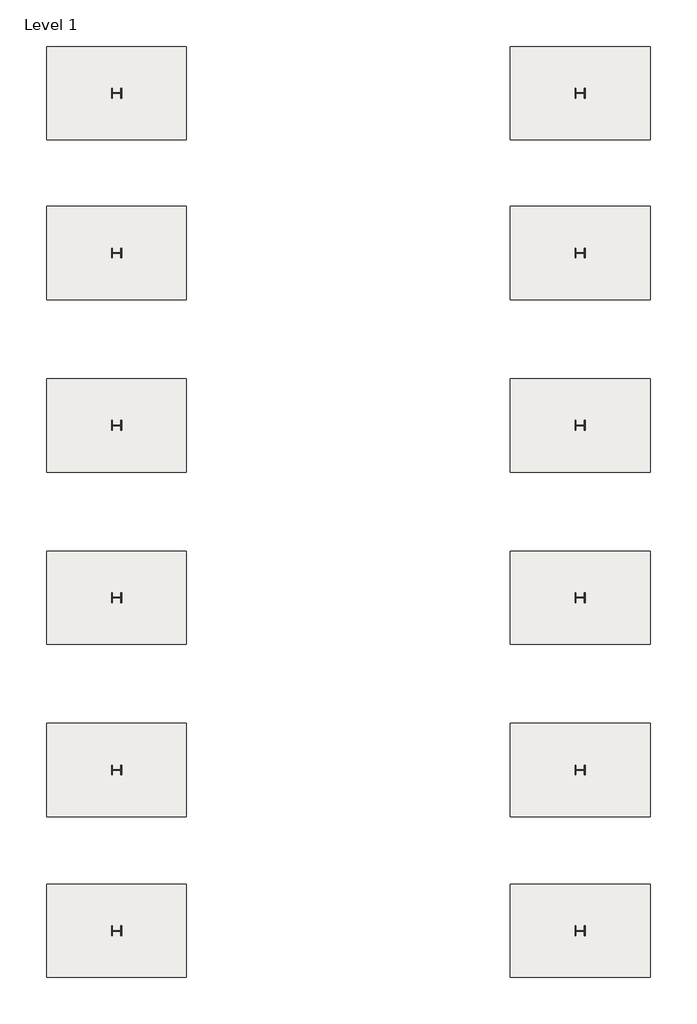
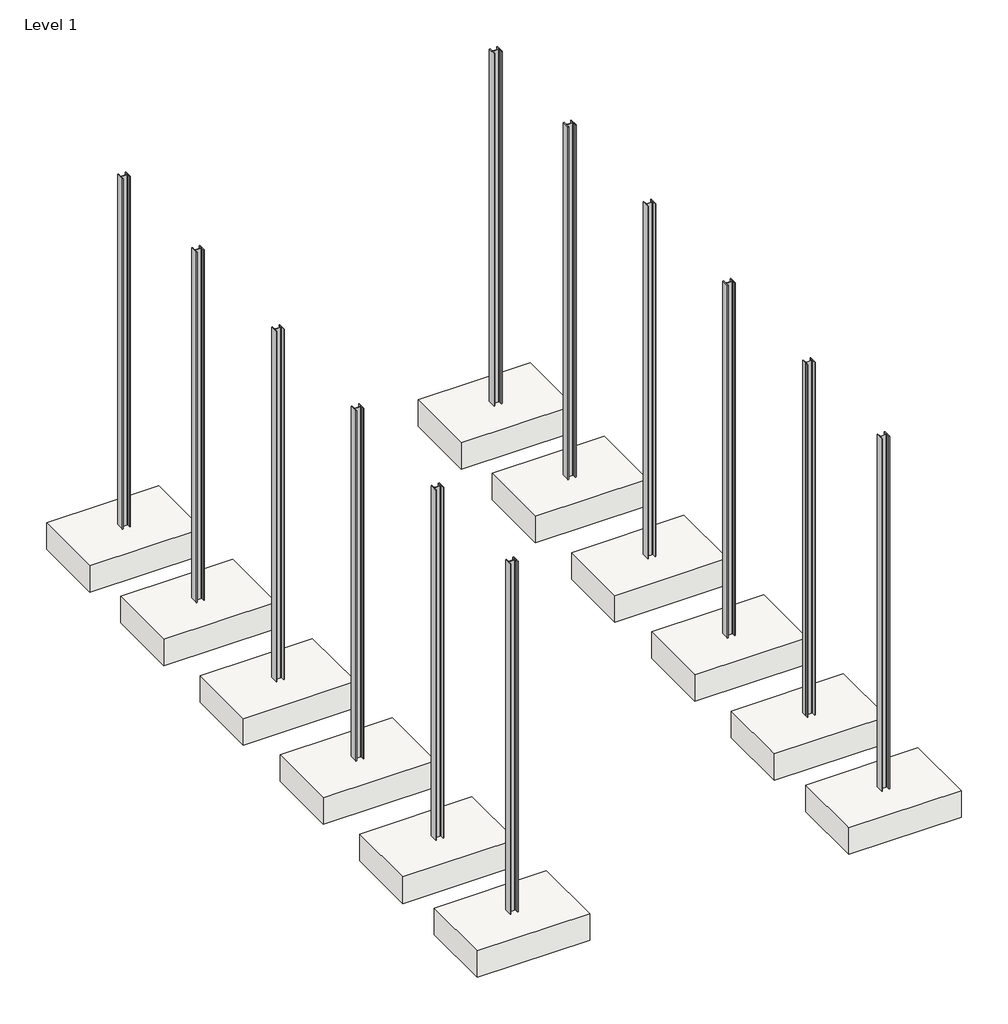
# One storey: 12 columns, 12 slabs.
"""IFC4 building model written with IfcOpenShell, lengths in millimetres."""

import ifcopenshell
import ifcopenshell.guid

model = None  # the IFC model being written
_history = None  # IfcOwnerHistory: only IFC2X3 demands one
_inside = {}  # id of a spatial element -> (the spatial element, [elements in it])
_under = {}  # id of a project, library or spatial element -> (it, [spatial elements below it])
_declared = {}  # id of a project -> (the project, [libraries it declares])
_typed = {}  # id of a type object -> (the type object, [elements of that type])
_made_of = {}  # id of a material, layer set ... -> (it, [elements and type objects made of it])


def new_model(schema):
    """Start an empty IFC model of exactly this schema.

    Asked for "IFC4X3", IfcOpenShell would pick the latest addendum, in which some entities
    have other attributes; the version numbers below select the first issue.
    IFC2X3 requires an IfcOwnerHistory on every rooted entity: one is made here for all.
    """
    global model, _history
    if schema == "IFC4X3":
        model = ifcopenshell.file(schema_version=(4, 3, 0, 0))
    else:
        model = ifcopenshell.file(schema=schema)
    _inside.clear()
    _under.clear()
    _declared.clear()
    _typed.clear()
    _made_of.clear()
    _history = None
    if model.schema == "IFC2X3":
        org = make("IfcOrganization", Name="unknown")
        user = make(
            "IfcPersonAndOrganization",
            ThePerson=make("IfcPerson", FamilyName="unknown"),
            TheOrganization=org,
        )
        app = make(
            "IfcApplication",
            ApplicationDeveloper=org,
            Version="unknown",
            ApplicationFullName="unknown",
            ApplicationIdentifier="unknown",
        )
        _history = make(
            "IfcOwnerHistory",
            OwningUser=user,
            OwningApplication=app,
            ChangeAction="ADDED",
            CreationDate=0,
        )
    return model


def make(cls, **values):
    """One entity of the class cls with the attributes given. An attribute that is None is left unset."""
    return model.create_entity(
        cls, **{name: value for name, value in values.items() if value is not None}
    )


def rooted(cls, **values):
    """An entity with a GlobalId (a new one), such as an element, a storey or a relation."""
    return make(cls, GlobalId=ifcopenshell.guid.new(), OwnerHistory=_history, **values)


def si_unit(unit_type, name, prefix=None):
    """IfcSIUnit, for example si_unit("LENGTHUNIT", "METRE", prefix="MILLI")."""
    return make("IfcSIUnit", UnitType=unit_type, Prefix=prefix, Name=name)


def assignment(units):
    """IfcUnitAssignment: the units of a project."""
    return None if units is None else make("IfcUnitAssignment", Units=units)


def point(xyz):
    """IfcCartesianPoint."""
    return None if xyz is None else make("IfcCartesianPoint", Coordinates=xyz)


def direction(xyz):
    """IfcDirection."""
    return None if xyz is None else make("IfcDirection", DirectionRatios=xyz)


def frame(location, z_axis=None, x_axis=None):
    """IfcAxis2Placement3D, a coordinate frame: its origin and axes. An axis left out is left unset."""
    return make(
        "IfcAxis2Placement3D",
        Location=point(location),
        Axis=direction(z_axis),
        RefDirection=direction(x_axis),
    )


def frame_2d(location, x_axis=None):
    """IfcAxis2Placement2D, a coordinate frame in the plane: its origin and x axis."""
    return make(
        "IfcAxis2Placement2D", Location=point(location), RefDirection=direction(x_axis)
    )


def origin():
    """The frame at (0, 0, 0) with its axes left unset."""
    return frame((0.0, 0.0, 0.0))


def place(relative_to, where):
    """IfcLocalPlacement: puts the frame where relative to a parent placement (None: the world)."""
    return make(
        "IfcLocalPlacement", PlacementRelTo=relative_to, RelativePlacement=where
    )


def context(
    kind, dimensions, precision=None, world=None, true_north=None, identifier=None
):
    """IfcGeometricRepresentationContext, for example the 3D "Model" context."""
    return make(
        "IfcGeometricRepresentationContext",
        ContextIdentifier=identifier,
        ContextType=kind,
        CoordinateSpaceDimension=dimensions,
        Precision=precision,
        WorldCoordinateSystem=world,
        TrueNorth=true_north,
    )


def project(units=None, contexts=None):
    """IfcProject with its units and contexts."""
    return rooted(
        "IfcProject",
        Name="project",
        RepresentationContexts=contexts,
        UnitsInContext=assignment(units),
    )


def spatial(cls, under=None, at=None, **own):
    """A site, building, storey or space (cls), placed at a placement, below another one or the project."""
    s = rooted(cls, ObjectPlacement=at, **own)
    if under is not None:
        _under.setdefault(under.id(), (under, []))[1].append(s)
    return s


def polyline(points):
    """IfcPolyline through the points."""
    return make("IfcPolyline", Points=[point(p) for p in points])


def circle_curve(where, radius):
    """IfcCircle in the frame where."""
    return make("IfcCircle", Position=where, Radius=radius)


def trimmed(basis, trim1, trim2, sense, master):
    """IfcTrimmedCurve: the piece of a basis curve between two trims."""
    return make(
        "IfcTrimmedCurve",
        BasisCurve=basis,
        Trim1=trim1,
        Trim2=trim2,
        SenseAgreement=sense,
        MasterRepresentation=master,
    )


def segment(curve, same_sense, transition):
    """IfcCompositeCurveSegment."""
    return make(
        "IfcCompositeCurveSegment",
        Transition=transition,
        SameSense=same_sense,
        ParentCurve=curve,
    )


def composite_curve(segments, self_intersect=None):
    """IfcCompositeCurve: segments joined end to end."""
    return make("IfcCompositeCurve", Segments=segments, SelfIntersect=self_intersect)


def outline(outer, holes=None, kind="AREA"):
    """IfcArbitraryClosedProfileDef: a profile drawn as a closed curve; with holes, ...WithVoids."""
    if holes is None:
        return make("IfcArbitraryClosedProfileDef", ProfileType=kind, OuterCurve=outer)
    return make(
        "IfcArbitraryProfileDefWithVoids",
        ProfileType=kind,
        OuterCurve=outer,
        InnerCurves=holes,
    )


def extrude(swept, where, along, depth):
    """IfcExtrudedAreaSolid: the profile swept, set in the frame where, extruded along a direction by depth."""
    return make(
        "IfcExtrudedAreaSolid",
        SweptArea=swept,
        Position=where,
        ExtrudedDirection=direction(along),
        Depth=depth,
    )


def shape(context_of_items, identifier, shape_type, items):
    """IfcShapeRepresentation: the items that make up one representation, for example the "Body"."""
    return make(
        "IfcShapeRepresentation",
        ContextOfItems=context_of_items,
        RepresentationIdentifier=identifier,
        RepresentationType=shape_type,
        Items=items,
    )


def source(mapping_origin, context_of_items, identifier, shape_type, items):
    """IfcRepresentationMap: a shape defined once, which mapped items show again and again."""
    return make(
        "IfcRepresentationMap",
        MappingOrigin=mapping_origin,
        MappedRepresentation=shape(context_of_items, identifier, shape_type, items),
    )


def transform(
    local_origin,
    x_axis=None,
    y_axis=None,
    z_axis=None,
    scale=None,
    scale2=None,
    scale3=None,
    uniform=True,
):
    """IfcCartesianTransformationOperator3D, or its non-uniform kind. x_axis, y_axis, z_axis: its Axis1, 2, 3."""
    if uniform:
        return make(
            "IfcCartesianTransformationOperator3D",
            Axis1=direction(x_axis),
            Axis2=direction(y_axis),
            LocalOrigin=point(local_origin),
            Scale=scale,
            Axis3=direction(z_axis),
        )
    return make(
        "IfcCartesianTransformationOperator3DnonUniform",
        Axis1=direction(x_axis),
        Axis2=direction(y_axis),
        LocalOrigin=point(local_origin),
        Scale=scale,
        Axis3=direction(z_axis),
        Scale2=scale2,
        Scale3=scale3,
    )


def mapped(mapping_source, mapping_target):
    """IfcMappedItem: shows the shape of a source again, moved by a transform."""
    return make(
        "IfcMappedItem", MappingSource=mapping_source, MappingTarget=mapping_target
    )


def made_of(thing, what):
    """Note that an element or type object is made of a material, layer set ...; save() writes the relation."""
    if what is not None:
        _made_of.setdefault(what.id(), (what, []))[1].append(thing)
    return thing


def element(
    cls,
    number,
    at=None,
    inside=None,
    cuts=None,
    type_object=None,
    material=None,
    context=None,
    identifier="Body",
    shape_type=None,
    held_by="IfcProductDefinitionShape",
    body=None,
    shapes=None,
    **own,
):
    """One element of the class cls, such as IfcWall. Its Tag is "e" and its number.

    at: its placement. inside: the storey or other place that contains it. cuts: it is an
    opening in that element (IfcRelVoidsElement). A single representation is given by context,
    identifier, shape_type and body (its items); several are given by shapes. held_by: the class
    of the entity that holds the representations. save() writes the other relations.
    """
    e = rooted(cls, Tag="e%d" % number, ObjectPlacement=at, **own)
    if body is not None:
        shapes = [shape(context, identifier, shape_type, body)]
    if shapes is not None:
        e.Representation = make(held_by, Representations=shapes)
    if inside is not None:
        _inside.setdefault(inside.id(), (inside, []))[1].append(e)
    if cuts is not None:
        rooted(
            "IfcRelVoidsElement", RelatingBuildingElement=cuts, RelatedOpeningElement=e
        )
    if type_object is not None:
        _typed.setdefault(type_object.id(), (type_object, []))[1].append(e)
    return made_of(e, material)


def aggregate(whole, parts):
    """IfcRelAggregates: a whole, such as a stair, and the parts it consists of."""
    return rooted("IfcRelAggregates", RelatingObject=whole, RelatedObjects=parts)


def save(model, path):
    """Write the relations noted so far, then the file.

    IfcRelAggregates (storeys below a building ...), IfcRelContainedInSpatialStructure (elements
    in a storey), IfcRelDefinesByType, IfcRelAssociatesMaterial and IfcRelDeclares: one each for
    every whole, place, type object, material and project.
    """
    for whole, parts in _under.values():
        aggregate(whole, parts)
    for where, things in _inside.values():
        rooted(
            "IfcRelContainedInSpatialStructure",
            RelatedElements=things,
            RelatingStructure=where,
        )
    for kind, things in _typed.values():
        rooted("IfcRelDefinesByType", RelatedObjects=things, RelatingType=kind)
    for what, things in _made_of.values():
        rooted("IfcRelAssociatesMaterial", RelatedObjects=things, RelatingMaterial=what)
    for by, libraries in _declared.values():
        rooted("IfcRelDeclares", RelatingContext=by, RelatedDefinitions=libraries)
    model.write(path)


def slab_5ba74754(model_context):
    return source(origin(), model_context, "Body", "SweptSolid", [
        extrude(outline(polyline([(609.6, 914.4), (609.6, -914.4), (-609.6, -914.4), (-609.6, 914.4), (609.6, 914.4)])), frame((0.0, 0.0, -457.2), z_axis=(0.0, 0.0, 1.0), x_axis=(1.0, 0.0, 0.0)), (0.0, 0.0, 1.0), 457.2),
    ])


model = new_model("IFC4")

# Units and contexts
model_context = context("Model", 3, world=origin())
ifc_project = project(units=[si_unit("LENGTHUNIT", "METRE", prefix="MILLI")], contexts=[model_context])

# Site, building, storey
site = spatial("IfcSite", under=ifc_project)
building = spatial("IfcBuilding", under=site)
storey = spatial("IfcBuildingStorey", under=building, Name="Level 1", Elevation=0.0)

# Columns
placement = place(None, origin())
element("IfcColumn", 1, ObjectType="W-Wide Flange-Column : W5X19", at=placement, inside=storey, context=model_context, shape_type="SweptSolid", body=[
    extrude(outline(composite_curve([segment(polyline([(-222.2451664, 2315.5517583), (-211.3231664, 2315.5517583), (-211.3231664, 2264.8152583)]), True, "CONTINUOUS"), segment(trimmed(circle_curve(frame_2d((-201.6076664, 2264.8152583)), 9.7155), [point((-211.3231664, 2264.8152583))], [point((-201.6076664, 2255.0997583))], True, "CARTESIAN"), True, "CONTINUOUS"), segment(polyline([(-201.6076664, 2255.0997583), (-112.0726664, 2255.0997583)]), True, "CONTINUOUS"), segment(trimmed(circle_curve(frame_2d((-112.0726664, 2264.8152583)), 9.7155), [point((-112.0726664, 2255.0997583))], [point((-102.3571664, 2264.8152583))], True, "CARTESIAN"), True, "CONTINUOUS"), segment(polyline([(-102.3571664, 2264.8152583), (-102.3571664, 2315.5517583), (-91.4351664, 2315.5517583), (-91.4351664, 2187.7897583), (-102.3571664, 2187.7897583), (-102.3571664, 2238.5262583)]), True, "CONTINUOUS"), segment(trimmed(circle_curve(frame_2d((-112.0726664, 2238.5262583)), 9.7155), [point((-102.3571664, 2238.5262583))], [point((-112.0726664, 2248.2417583))], True, "CARTESIAN"), True, "CONTINUOUS"), segment(polyline([(-112.0726664, 2248.2417583), (-201.6076664, 2248.2417583)]), True, "CONTINUOUS"), segment(trimmed(circle_curve(frame_2d((-201.6076664, 2238.5262583)), 9.7155), [point((-201.6076664, 2248.2417583))], [point((-211.3231664, 2238.5262583))], True, "CARTESIAN"), True, "CONTINUOUS"), segment(polyline([(-211.3231664, 2238.5262583), (-211.3231664, 2187.7897583), (-222.2451664, 2187.7897583), (-222.2451664, 2315.5517583)]), True, "CONTINUOUS")], self_intersect=False)), frame((0.0, 0.0, -304.8), z_axis=(0.0, 0.0, 1.0), x_axis=(1.0, 0.0, 0.0)), (0.0, 0.0, 1.0), 6079.1336143),
])
element("IfcColumn", 2, ObjectType="W-Wide Flange-Column : W5X19", at=placement, inside=storey, context=model_context, shape_type="SweptSolid", body=[
    extrude(outline(composite_curve([segment(polyline([(-6280.1451664, 2315.5517583), (-6269.2231664, 2315.5517583), (-6269.2231664, 2264.8152583)]), True, "CONTINUOUS"), segment(trimmed(circle_curve(frame_2d((-6259.5076664, 2264.8152583)), 9.7155), [point((-6269.2231664, 2264.8152583))], [point((-6259.5076664, 2255.0997583))], True, "CARTESIAN"), True, "CONTINUOUS"), segment(polyline([(-6259.5076664, 2255.0997583), (-6169.9726664, 2255.0997583)]), True, "CONTINUOUS"), segment(trimmed(circle_curve(frame_2d((-6169.9726664, 2264.8152583)), 9.7155), [point((-6169.9726664, 2255.0997583))], [point((-6160.2571664, 2264.8152583))], True, "CARTESIAN"), True, "CONTINUOUS"), segment(polyline([(-6160.2571664, 2264.8152583), (-6160.2571664, 2315.5517583), (-6149.3351664, 2315.5517583), (-6149.3351664, 2187.7897583), (-6160.2571664, 2187.7897583), (-6160.2571664, 2238.5262583)]), True, "CONTINUOUS"), segment(trimmed(circle_curve(frame_2d((-6169.9726664, 2238.5262583)), 9.7155), [point((-6160.2571664, 2238.5262583))], [point((-6169.9726664, 2248.2417583))], True, "CARTESIAN"), True, "CONTINUOUS"), segment(polyline([(-6169.9726664, 2248.2417583), (-6259.5076664, 2248.2417583)]), True, "CONTINUOUS"), segment(trimmed(circle_curve(frame_2d((-6259.5076664, 2238.5262583)), 9.7155), [point((-6259.5076664, 2248.2417583))], [point((-6269.2231664, 2238.5262583))], True, "CARTESIAN"), True, "CONTINUOUS"), segment(polyline([(-6269.2231664, 2238.5262583), (-6269.2231664, 2187.7897583), (-6280.1451664, 2187.7897583), (-6280.1451664, 2315.5517583)]), True, "CONTINUOUS")], self_intersect=False)), frame((0.0, 0.0, -304.8), z_axis=(0.0, 0.0, 1.0), x_axis=(1.0, 0.0, 0.0)), (0.0, 0.0, 1.0), 6040.3114063),
])
element("IfcColumn", 3, ObjectType="W-Wide Flange-Column : W5X19", at=placement, inside=storey, context=model_context, shape_type="SweptSolid", body=[
    extrude(outline(composite_curve([segment(polyline([(-222.2451664, 4567.4626058), (-211.3231664, 4567.4626058), (-211.3231664, 4516.7261058)]), True, "CONTINUOUS"), segment(trimmed(circle_curve(frame_2d((-201.6076664, 4516.7261058)), 9.7155), [point((-211.3231664, 4516.7261058))], [point((-201.6076664, 4507.0106058))], True, "CARTESIAN"), True, "CONTINUOUS"), segment(polyline([(-201.6076664, 4507.0106058), (-112.0726664, 4507.0106058)]), True, "CONTINUOUS"), segment(trimmed(circle_curve(frame_2d((-112.0726664, 4516.7261058)), 9.7155), [point((-112.0726664, 4507.0106058))], [point((-102.3571664, 4516.7261058))], True, "CARTESIAN"), True, "CONTINUOUS"), segment(polyline([(-102.3571664, 4516.7261058), (-102.3571664, 4567.4626058), (-91.4351664, 4567.4626058), (-91.4351664, 4439.7006058), (-102.3571664, 4439.7006058), (-102.3571664, 4490.4371058)]), True, "CONTINUOUS"), segment(trimmed(circle_curve(frame_2d((-112.0726664, 4490.4371058)), 9.7155), [point((-102.3571664, 4490.4371058))], [point((-112.0726664, 4500.1526058))], True, "CARTESIAN"), True, "CONTINUOUS"), segment(polyline([(-112.0726664, 4500.1526058), (-201.6076664, 4500.1526058)]), True, "CONTINUOUS"), segment(trimmed(circle_curve(frame_2d((-201.6076664, 4490.4371058)), 9.7155), [point((-201.6076664, 4500.1526058))], [point((-211.3231664, 4490.4371058))], True, "CARTESIAN"), True, "CONTINUOUS"), segment(polyline([(-211.3231664, 4490.4371058), (-211.3231664, 4439.7006058), (-222.2451664, 4439.7006058), (-222.2451664, 4567.4626058)]), True, "CONTINUOUS")], self_intersect=False)), frame((0.0, 0.0, -304.8), z_axis=(0.0, 0.0, 1.0), x_axis=(1.0, 0.0, 0.0)), (0.0, 0.0, 1.0), 6079.1336143),
])
element("IfcColumn", 4, ObjectType="W-Wide Flange-Column : W5X19", at=placement, inside=storey, context=model_context, shape_type="SweptSolid", body=[
    extrude(outline(composite_curve([segment(polyline([(-6280.1451664, 4567.4626058), (-6269.2231664, 4567.4626058), (-6269.2231664, 4516.7261058)]), True, "CONTINUOUS"), segment(trimmed(circle_curve(frame_2d((-6259.5076664, 4516.7261058)), 9.7155), [point((-6269.2231664, 4516.7261058))], [point((-6259.5076664, 4507.0106058))], True, "CARTESIAN"), True, "CONTINUOUS"), segment(polyline([(-6259.5076664, 4507.0106058), (-6169.9726664, 4507.0106058)]), True, "CONTINUOUS"), segment(trimmed(circle_curve(frame_2d((-6169.9726664, 4516.7261058)), 9.7155), [point((-6169.9726664, 4507.0106058))], [point((-6160.2571664, 4516.7261058))], True, "CARTESIAN"), True, "CONTINUOUS"), segment(polyline([(-6160.2571664, 4516.7261058), (-6160.2571664, 4567.4626058), (-6149.3351664, 4567.4626058), (-6149.3351664, 4439.7006058), (-6160.2571664, 4439.7006058), (-6160.2571664, 4490.4371058)]), True, "CONTINUOUS"), segment(trimmed(circle_curve(frame_2d((-6169.9726664, 4490.4371058)), 9.7155), [point((-6160.2571664, 4490.4371058))], [point((-6169.9726664, 4500.1526058))], True, "CARTESIAN"), True, "CONTINUOUS"), segment(polyline([(-6169.9726664, 4500.1526058), (-6259.5076664, 4500.1526058)]), True, "CONTINUOUS"), segment(trimmed(circle_curve(frame_2d((-6259.5076664, 4490.4371058)), 9.7155), [point((-6259.5076664, 4500.1526058))], [point((-6269.2231664, 4490.4371058))], True, "CARTESIAN"), True, "CONTINUOUS"), segment(polyline([(-6269.2231664, 4490.4371058), (-6269.2231664, 4439.7006058), (-6280.1451664, 4439.7006058), (-6280.1451664, 4567.4626058)]), True, "CONTINUOUS")], self_intersect=False)), frame((0.0, 0.0, -304.8), z_axis=(0.0, 0.0, 1.0), x_axis=(1.0, 0.0, 0.0)), (0.0, 0.0, 1.0), 6040.3114063),
])
element("IfcColumn", 5, ObjectType="W-Wide Flange-Column : W5X19", at=placement, inside=storey, context=model_context, shape_type="SweptSolid", body=[
    extrude(outline(composite_curve([segment(polyline([(-222.2451664, 6819.3734532), (-211.3231664, 6819.3734532), (-211.3231664, 6768.6369532)]), True, "CONTINUOUS"), segment(trimmed(circle_curve(frame_2d((-201.6076664, 6768.6369532)), 9.7155), [point((-211.3231664, 6768.6369532))], [point((-201.6076664, 6758.9214532))], True, "CARTESIAN"), True, "CONTINUOUS"), segment(polyline([(-201.6076664, 6758.9214532), (-112.0726664, 6758.9214532)]), True, "CONTINUOUS"), segment(trimmed(circle_curve(frame_2d((-112.0726664, 6768.6369532)), 9.7155), [point((-112.0726664, 6758.9214532))], [point((-102.3571664, 6768.6369532))], True, "CARTESIAN"), True, "CONTINUOUS"), segment(polyline([(-102.3571664, 6768.6369532), (-102.3571664, 6819.3734532), (-91.4351664, 6819.3734532), (-91.4351664, 6691.6114532), (-102.3571664, 6691.6114532), (-102.3571664, 6742.3479532)]), True, "CONTINUOUS"), segment(trimmed(circle_curve(frame_2d((-112.0726664, 6742.3479532)), 9.7155), [point((-102.3571664, 6742.3479532))], [point((-112.0726664, 6752.0634532))], True, "CARTESIAN"), True, "CONTINUOUS"), segment(polyline([(-112.0726664, 6752.0634532), (-201.6076664, 6752.0634532)]), True, "CONTINUOUS"), segment(trimmed(circle_curve(frame_2d((-201.6076664, 6742.3479532)), 9.7155), [point((-201.6076664, 6752.0634532))], [point((-211.3231664, 6742.3479532))], True, "CARTESIAN"), True, "CONTINUOUS"), segment(polyline([(-211.3231664, 6742.3479532), (-211.3231664, 6691.6114532), (-222.2451664, 6691.6114532), (-222.2451664, 6819.3734532)]), True, "CONTINUOUS")], self_intersect=False)), frame((0.0, 0.0, -304.8), z_axis=(0.0, 0.0, 1.0), x_axis=(1.0, 0.0, 0.0)), (0.0, 0.0, 1.0), 6079.1336143),
])
element("IfcColumn", 6, ObjectType="W-Wide Flange-Column : W5X19", at=placement, inside=storey, context=model_context, shape_type="SweptSolid", body=[
    extrude(outline(composite_curve([segment(polyline([(-6280.1451664, 6819.3734532), (-6269.2231664, 6819.3734532), (-6269.2231664, 6768.6369532)]), True, "CONTINUOUS"), segment(trimmed(circle_curve(frame_2d((-6259.5076664, 6768.6369532)), 9.7155), [point((-6269.2231664, 6768.6369532))], [point((-6259.5076664, 6758.9214532))], True, "CARTESIAN"), True, "CONTINUOUS"), segment(polyline([(-6259.5076664, 6758.9214532), (-6169.9726664, 6758.9214532)]), True, "CONTINUOUS"), segment(trimmed(circle_curve(frame_2d((-6169.9726664, 6768.6369532)), 9.7155), [point((-6169.9726664, 6758.9214532))], [point((-6160.2571664, 6768.6369532))], True, "CARTESIAN"), True, "CONTINUOUS"), segment(polyline([(-6160.2571664, 6768.6369532), (-6160.2571664, 6819.3734532), (-6149.3351664, 6819.3734532), (-6149.3351664, 6691.6114532), (-6160.2571664, 6691.6114532), (-6160.2571664, 6742.3479532)]), True, "CONTINUOUS"), segment(trimmed(circle_curve(frame_2d((-6169.9726664, 6742.3479532)), 9.7155), [point((-6160.2571664, 6742.3479532))], [point((-6169.9726664, 6752.0634532))], True, "CARTESIAN"), True, "CONTINUOUS"), segment(polyline([(-6169.9726664, 6752.0634532), (-6259.5076664, 6752.0634532)]), True, "CONTINUOUS"), segment(trimmed(circle_curve(frame_2d((-6259.5076664, 6742.3479532)), 9.7155), [point((-6259.5076664, 6752.0634532))], [point((-6269.2231664, 6742.3479532))], True, "CARTESIAN"), True, "CONTINUOUS"), segment(polyline([(-6269.2231664, 6742.3479532), (-6269.2231664, 6691.6114532), (-6280.1451664, 6691.6114532), (-6280.1451664, 6819.3734532)]), True, "CONTINUOUS")], self_intersect=False)), frame((0.0, 0.0, -304.8), z_axis=(0.0, 0.0, 1.0), x_axis=(1.0, 0.0, 0.0)), (0.0, 0.0, 1.0), 6040.3114063),
])
element("IfcColumn", 7, ObjectType="W-Wide Flange-Column : W5X19", at=placement, inside=storey, context=model_context, shape_type="SweptSolid", body=[
    extrude(outline(composite_curve([segment(polyline([(-222.2451664, 9071.2843006), (-211.3231664, 9071.2843006), (-211.3231664, 9020.5478006)]), True, "CONTINUOUS"), segment(trimmed(circle_curve(frame_2d((-201.6076664, 9020.5478006)), 9.7155), [point((-211.3231664, 9020.5478006))], [point((-201.6076664, 9010.8323006))], True, "CARTESIAN"), True, "CONTINUOUS"), segment(polyline([(-201.6076664, 9010.8323006), (-112.0726664, 9010.8323006)]), True, "CONTINUOUS"), segment(trimmed(circle_curve(frame_2d((-112.0726664, 9020.5478006)), 9.7155), [point((-112.0726664, 9010.8323006))], [point((-102.3571664, 9020.5478006))], True, "CARTESIAN"), True, "CONTINUOUS"), segment(polyline([(-102.3571664, 9020.5478006), (-102.3571664, 9071.2843006), (-91.4351664, 9071.2843006), (-91.4351664, 8943.5223006), (-102.3571664, 8943.5223006), (-102.3571664, 8994.2588006)]), True, "CONTINUOUS"), segment(trimmed(circle_curve(frame_2d((-112.0726664, 8994.2588006)), 9.7155), [point((-102.3571664, 8994.2588006))], [point((-112.0726664, 9003.9743006))], True, "CARTESIAN"), True, "CONTINUOUS"), segment(polyline([(-112.0726664, 9003.9743006), (-201.6076664, 9003.9743006)]), True, "CONTINUOUS"), segment(trimmed(circle_curve(frame_2d((-201.6076664, 8994.2588006)), 9.7155), [point((-201.6076664, 9003.9743006))], [point((-211.3231664, 8994.2588006))], True, "CARTESIAN"), True, "CONTINUOUS"), segment(polyline([(-211.3231664, 8994.2588006), (-211.3231664, 8943.5223006), (-222.2451664, 8943.5223006), (-222.2451664, 9071.2843006)]), True, "CONTINUOUS")], self_intersect=False)), frame((0.0, 0.0, -304.8), z_axis=(0.0, 0.0, 1.0), x_axis=(1.0, 0.0, 0.0)), (0.0, 0.0, 1.0), 6079.1336143),
])
element("IfcColumn", 8, ObjectType="W-Wide Flange-Column : W5X19", at=placement, inside=storey, context=model_context, shape_type="SweptSolid", body=[
    extrude(outline(composite_curve([segment(polyline([(-6280.1451664, 9071.2843006), (-6269.2231664, 9071.2843006), (-6269.2231664, 9020.5478006)]), True, "CONTINUOUS"), segment(trimmed(circle_curve(frame_2d((-6259.5076664, 9020.5478006)), 9.7155), [point((-6269.2231664, 9020.5478006))], [point((-6259.5076664, 9010.8323006))], True, "CARTESIAN"), True, "CONTINUOUS"), segment(polyline([(-6259.5076664, 9010.8323006), (-6169.9726664, 9010.8323006)]), True, "CONTINUOUS"), segment(trimmed(circle_curve(frame_2d((-6169.9726664, 9020.5478006)), 9.7155), [point((-6169.9726664, 9010.8323006))], [point((-6160.2571664, 9020.5478006))], True, "CARTESIAN"), True, "CONTINUOUS"), segment(polyline([(-6160.2571664, 9020.5478006), (-6160.2571664, 9071.2843006), (-6149.3351664, 9071.2843006), (-6149.3351664, 8943.5223006), (-6160.2571664, 8943.5223006), (-6160.2571664, 8994.2588006)]), True, "CONTINUOUS"), segment(trimmed(circle_curve(frame_2d((-6169.9726664, 8994.2588006)), 9.7155), [point((-6160.2571664, 8994.2588006))], [point((-6169.9726664, 9003.9743006))], True, "CARTESIAN"), True, "CONTINUOUS"), segment(polyline([(-6169.9726664, 9003.9743006), (-6259.5076664, 9003.9743006)]), True, "CONTINUOUS"), segment(trimmed(circle_curve(frame_2d((-6259.5076664, 8994.2588006)), 9.7155), [point((-6259.5076664, 9003.9743006))], [point((-6269.2231664, 8994.2588006))], True, "CARTESIAN"), True, "CONTINUOUS"), segment(polyline([(-6269.2231664, 8994.2588006), (-6269.2231664, 8943.5223006), (-6280.1451664, 8943.5223006), (-6280.1451664, 9071.2843006)]), True, "CONTINUOUS")], self_intersect=False)), frame((0.0, 0.0, -304.8), z_axis=(0.0, 0.0, 1.0), x_axis=(1.0, 0.0, 0.0)), (0.0, 0.0, 1.0), 6040.3114063),
])
element("IfcColumn", 9, ObjectType="W-Wide Flange-Column : W5X19", at=placement, inside=storey, context=model_context, shape_type="SweptSolid", body=[
    extrude(outline(composite_curve([segment(polyline([(-222.2451664, 11160.4343006), (-211.3231664, 11160.4343006), (-211.3231664, 11109.6978006)]), True, "CONTINUOUS"), segment(trimmed(circle_curve(frame_2d((-201.6076664, 11109.6978006)), 9.7155), [point((-211.3231664, 11109.6978006))], [point((-201.6076664, 11099.9823006))], True, "CARTESIAN"), True, "CONTINUOUS"), segment(polyline([(-201.6076664, 11099.9823006), (-112.0726664, 11099.9823006)]), True, "CONTINUOUS"), segment(trimmed(circle_curve(frame_2d((-112.0726664, 11109.6978006)), 9.7155), [point((-112.0726664, 11099.9823006))], [point((-102.3571664, 11109.6978006))], True, "CARTESIAN"), True, "CONTINUOUS"), segment(polyline([(-102.3571664, 11109.6978006), (-102.3571664, 11160.4343006), (-91.4351664, 11160.4343006), (-91.4351664, 11032.6723006), (-102.3571664, 11032.6723006), (-102.3571664, 11083.4088006)]), True, "CONTINUOUS"), segment(trimmed(circle_curve(frame_2d((-112.0726664, 11083.4088006)), 9.7155), [point((-102.3571664, 11083.4088006))], [point((-112.0726664, 11093.1243006))], True, "CARTESIAN"), True, "CONTINUOUS"), segment(polyline([(-112.0726664, 11093.1243006), (-201.6076664, 11093.1243006)]), True, "CONTINUOUS"), segment(trimmed(circle_curve(frame_2d((-201.6076664, 11083.4088006)), 9.7155), [point((-201.6076664, 11093.1243006))], [point((-211.3231664, 11083.4088006))], True, "CARTESIAN"), True, "CONTINUOUS"), segment(polyline([(-211.3231664, 11083.4088006), (-211.3231664, 11032.6723006), (-222.2451664, 11032.6723006), (-222.2451664, 11160.4343006)]), True, "CONTINUOUS")], self_intersect=False)), frame((0.0, 0.0, -304.8), z_axis=(0.0, 0.0, 1.0), x_axis=(1.0, 0.0, 0.0)), (0.0, 0.0, 1.0), 6079.1336143),
])
element("IfcColumn", 10, ObjectType="W-Wide Flange-Column : W5X19", at=placement, inside=storey, context=model_context, shape_type="SweptSolid", body=[
    extrude(outline(composite_curve([segment(polyline([(-6280.1451664, 11160.4343006), (-6269.2231664, 11160.4343006), (-6269.2231664, 11109.6978006)]), True, "CONTINUOUS"), segment(trimmed(circle_curve(frame_2d((-6259.5076664, 11109.6978006)), 9.7155), [point((-6269.2231664, 11109.6978006))], [point((-6259.5076664, 11099.9823006))], True, "CARTESIAN"), True, "CONTINUOUS"), segment(polyline([(-6259.5076664, 11099.9823006), (-6169.9726664, 11099.9823006)]), True, "CONTINUOUS"), segment(trimmed(circle_curve(frame_2d((-6169.9726664, 11109.6978006)), 9.7155), [point((-6169.9726664, 11099.9823006))], [point((-6160.2571664, 11109.6978006))], True, "CARTESIAN"), True, "CONTINUOUS"), segment(polyline([(-6160.2571664, 11109.6978006), (-6160.2571664, 11160.4343006), (-6149.3351664, 11160.4343006), (-6149.3351664, 11032.6723006), (-6160.2571664, 11032.6723006), (-6160.2571664, 11083.4088006)]), True, "CONTINUOUS"), segment(trimmed(circle_curve(frame_2d((-6169.9726664, 11083.4088006)), 9.7155), [point((-6160.2571664, 11083.4088006))], [point((-6169.9726664, 11093.1243006))], True, "CARTESIAN"), True, "CONTINUOUS"), segment(polyline([(-6169.9726664, 11093.1243006), (-6259.5076664, 11093.1243006)]), True, "CONTINUOUS"), segment(trimmed(circle_curve(frame_2d((-6259.5076664, 11083.4088006)), 9.7155), [point((-6259.5076664, 11093.1243006))], [point((-6269.2231664, 11083.4088006))], True, "CARTESIAN"), True, "CONTINUOUS"), segment(polyline([(-6269.2231664, 11083.4088006), (-6269.2231664, 11032.6723006), (-6280.1451664, 11032.6723006), (-6280.1451664, 11160.4343006)]), True, "CONTINUOUS")], self_intersect=False)), frame((0.0, 0.0, -304.8), z_axis=(0.0, 0.0, 1.0), x_axis=(1.0, 0.0, 0.0)), (0.0, 0.0, 1.0), 6040.3114063),
])
element("IfcColumn", 11, ObjectType="W-Wide Flange-Column : W5X19", at=placement, inside=storey, context=model_context, shape_type="SweptSolid", body=[
    extrude(outline(composite_curve([segment(polyline([(-222.2451664, 213.7017583), (-211.3231664, 213.7017583), (-211.3231664, 162.9652583)]), True, "CONTINUOUS"), segment(trimmed(circle_curve(frame_2d((-201.6076664, 162.9652583)), 9.7155), [point((-211.3231664, 162.9652583))], [point((-201.6076664, 153.2497583))], True, "CARTESIAN"), True, "CONTINUOUS"), segment(polyline([(-201.6076664, 153.2497583), (-112.0726664, 153.2497583)]), True, "CONTINUOUS"), segment(trimmed(circle_curve(frame_2d((-112.0726664, 162.9652583)), 9.7155), [point((-112.0726664, 153.2497583))], [point((-102.3571664, 162.9652583))], True, "CARTESIAN"), True, "CONTINUOUS"), segment(polyline([(-102.3571664, 162.9652583), (-102.3571664, 213.7017583), (-91.4351664, 213.7017583), (-91.4351664, 85.9397583), (-102.3571664, 85.9397583), (-102.3571664, 136.6762583)]), True, "CONTINUOUS"), segment(trimmed(circle_curve(frame_2d((-112.0726664, 136.6762583)), 9.7155), [point((-102.3571664, 136.6762583))], [point((-112.0726664, 146.3917583))], True, "CARTESIAN"), True, "CONTINUOUS"), segment(polyline([(-112.0726664, 146.3917583), (-201.6076664, 146.3917583)]), True, "CONTINUOUS"), segment(trimmed(circle_curve(frame_2d((-201.6076664, 136.6762583)), 9.7155), [point((-201.6076664, 146.3917583))], [point((-211.3231664, 136.6762583))], True, "CARTESIAN"), True, "CONTINUOUS"), segment(polyline([(-211.3231664, 136.6762583), (-211.3231664, 85.9397583), (-222.2451664, 85.9397583), (-222.2451664, 213.7017583)]), True, "CONTINUOUS")], self_intersect=False)), frame((0.0, 0.0, -304.8), z_axis=(0.0, 0.0, 1.0), x_axis=(1.0, 0.0, 0.0)), (0.0, 0.0, 1.0), 6079.1336143),
])
element("IfcColumn", 12, ObjectType="W-Wide Flange-Column : W5X19", at=placement, inside=storey, context=model_context, shape_type="SweptSolid", body=[
    extrude(outline(composite_curve([segment(polyline([(-6280.1451664, 213.7017583), (-6269.2231664, 213.7017583), (-6269.2231664, 162.9652583)]), True, "CONTINUOUS"), segment(trimmed(circle_curve(frame_2d((-6259.5076664, 162.9652583)), 9.7155), [point((-6269.2231664, 162.9652583))], [point((-6259.5076664, 153.2497583))], True, "CARTESIAN"), True, "CONTINUOUS"), segment(polyline([(-6259.5076664, 153.2497583), (-6169.9726664, 153.2497583)]), True, "CONTINUOUS"), segment(trimmed(circle_curve(frame_2d((-6169.9726664, 162.9652583)), 9.7155), [point((-6169.9726664, 153.2497583))], [point((-6160.2571664, 162.9652583))], True, "CARTESIAN"), True, "CONTINUOUS"), segment(polyline([(-6160.2571664, 162.9652583), (-6160.2571664, 213.7017583), (-6149.3351664, 213.7017583), (-6149.3351664, 85.9397583), (-6160.2571664, 85.9397583), (-6160.2571664, 136.6762583)]), True, "CONTINUOUS"), segment(trimmed(circle_curve(frame_2d((-6169.9726664, 136.6762583)), 9.7155), [point((-6160.2571664, 136.6762583))], [point((-6169.9726664, 146.3917583))], True, "CARTESIAN"), True, "CONTINUOUS"), segment(polyline([(-6169.9726664, 146.3917583), (-6259.5076664, 146.3917583)]), True, "CONTINUOUS"), segment(trimmed(circle_curve(frame_2d((-6259.5076664, 136.6762583)), 9.7155), [point((-6259.5076664, 146.3917583))], [point((-6269.2231664, 136.6762583))], True, "CARTESIAN"), True, "CONTINUOUS"), segment(polyline([(-6269.2231664, 136.6762583), (-6269.2231664, 85.9397583), (-6280.1451664, 85.9397583), (-6280.1451664, 213.7017583)]), True, "CONTINUOUS")], self_intersect=False)), frame((0.0, 0.0, -304.8), z_axis=(0.0, 0.0, 1.0), x_axis=(1.0, 0.0, 0.0)), (0.0, 0.0, 1.0), 6040.3114063),
])

# Slabs
slab_shape = slab_5ba74754(model_context)
element("IfcSlab", 13, ObjectType="Footing-Rectangular : 72\" x 48\" x 18\"", at=placement, inside=storey, context=model_context, shape_type="MappedRepresentation", body=[
    mapped(slab_shape, transform((-156.8401664, 2251.6707583, -304.8), x_axis=(0.0, 1.0, 0.0), y_axis=(-1.0, 0.0, 0.0), z_axis=(0.0, 0.0, 1.0))),
])
element("IfcSlab", 14, ObjectType="Footing-Rectangular : 72\" x 48\" x 18\"", at=placement, inside=storey, context=model_context, shape_type="MappedRepresentation", body=[
    mapped(slab_shape, transform((-6214.7401664, 2251.6707583, -304.8), x_axis=(0.0, 1.0, 0.0), y_axis=(-1.0, 0.0, 0.0), z_axis=(0.0, 0.0, 1.0))),
])
element("IfcSlab", 15, ObjectType="Footing-Rectangular : 72\" x 48\" x 18\"", at=placement, inside=storey, context=model_context, shape_type="MappedRepresentation", body=[
    mapped(slab_shape, transform((-156.8401664, 4503.5816058, -304.8), x_axis=(0.0, 1.0, 0.0), y_axis=(-1.0, 0.0, 0.0), z_axis=(0.0, 0.0, 1.0))),
])
element("IfcSlab", 16, ObjectType="Footing-Rectangular : 72\" x 48\" x 18\"", at=placement, inside=storey, context=model_context, shape_type="MappedRepresentation", body=[
    mapped(slab_shape, transform((-6214.7401664, 4503.5816058, -304.8), x_axis=(0.0, 1.0, 0.0), y_axis=(-1.0, 0.0, 0.0), z_axis=(0.0, 0.0, 1.0))),
])
element("IfcSlab", 17, ObjectType="Footing-Rectangular : 72\" x 48\" x 18\"", at=placement, inside=storey, context=model_context, shape_type="MappedRepresentation", body=[
    mapped(slab_shape, transform((-156.8401664, 6755.4924532, -304.8), x_axis=(0.0, 1.0, 0.0), y_axis=(-1.0, 0.0, 0.0), z_axis=(0.0, 0.0, 1.0))),
])
element("IfcSlab", 18, ObjectType="Footing-Rectangular : 72\" x 48\" x 18\"", at=placement, inside=storey, context=model_context, shape_type="MappedRepresentation", body=[
    mapped(slab_shape, transform((-6214.7401664, 6755.4924532, -304.8), x_axis=(0.0, 1.0, 0.0), y_axis=(-1.0, 0.0, 0.0), z_axis=(0.0, 0.0, 1.0))),
])
element("IfcSlab", 19, ObjectType="Footing-Rectangular : 72\" x 48\" x 18\"", at=placement, inside=storey, context=model_context, shape_type="MappedRepresentation", body=[
    mapped(slab_shape, transform((-156.8401664, 9007.4033006, -304.8), x_axis=(0.0, 1.0, 0.0), y_axis=(-1.0, 0.0, 0.0), z_axis=(0.0, 0.0, 1.0))),
])
element("IfcSlab", 20, ObjectType="Footing-Rectangular : 72\" x 48\" x 18\"", at=placement, inside=storey, context=model_context, shape_type="MappedRepresentation", body=[
    mapped(slab_shape, transform((-6214.7401664, 9007.4033006, -304.8), x_axis=(0.0, 1.0, 0.0), y_axis=(-1.0, 0.0, 0.0), z_axis=(0.0, 0.0, 1.0))),
])
element("IfcSlab", 21, ObjectType="Footing-Rectangular : 72\" x 48\" x 18\"", at=placement, inside=storey, context=model_context, shape_type="MappedRepresentation", body=[
    mapped(slab_shape, transform((-156.8401664, 11096.5533006, -304.8), x_axis=(0.0, 1.0, 0.0), y_axis=(-1.0, 0.0, 0.0), z_axis=(0.0, 0.0, 1.0))),
])
element("IfcSlab", 22, ObjectType="Footing-Rectangular : 72\" x 48\" x 18\"", at=placement, inside=storey, context=model_context, shape_type="MappedRepresentation", body=[
    mapped(slab_shape, transform((-6214.7401664, 11096.5533006, -304.8), x_axis=(0.0, 1.0, 0.0), y_axis=(-1.0, 0.0, 0.0), z_axis=(0.0, 0.0, 1.0))),
])
element("IfcSlab", 23, ObjectType="Footing-Rectangular : 72\" x 48\" x 18\"", at=placement, inside=storey, context=model_context, shape_type="MappedRepresentation", body=[
    mapped(slab_shape, transform((-156.8401664, 149.8207583, -304.8), x_axis=(0.0, 1.0, 0.0), y_axis=(-1.0, 0.0, 0.0), z_axis=(0.0, 0.0, 1.0))),
])
element("IfcSlab", 24, ObjectType="Footing-Rectangular : 72\" x 48\" x 18\"", at=placement, inside=storey, context=model_context, shape_type="MappedRepresentation", body=[
    mapped(slab_shape, transform((-6214.7401664, 149.8207583, -304.8), x_axis=(0.0, 1.0, 0.0), y_axis=(-1.0, 0.0, 0.0), z_axis=(0.0, 0.0, 1.0))),
])

save(model, "model.ifc")

# Revit data of these elements
# Project information
#   Project Issue Date = "Issue Date"
#   Project Status = "Project Status"
#   Client Name = "Owner"
#   Project Address = "Enter address here"
#   Project Name = "Project Name"
#   Project Number = "Project Number"
# Grids (mm)
#   "A": line (-6214.74, 12667.798) -> (-6214.74, -2435.314)
#   "B": line (-156.84, 12667.798) -> (-156.84, -2435.314)
#   "01": line (2491.424, 11096.553) -> (-7738.74, 11096.553)
#   "02": line (2491.424, 9007.403) -> (-7738.74, 9007.403)
#   "03": line (2491.424, 6755.492) -> (-7738.74, 6755.492)
#   "04": line (2491.424, 4503.582) -> (-7738.74, 4503.582)
#   "05": line (2491.424, 2251.671) -> (-7738.74, 2251.671)
#   "06": line (2491.424, 149.821) -> (-7738.74, 149.821)
# Type "W-Wide Flange-Column : W5X19"
#   Assembly Code = "B10"
#   W = 19
#   bf = 0' - 5.03"
#   d = 0' - 5.15"
#   k = 0' - 0 13/16"
#   kr = 0' - 0.3825"
#   tf = 0' - 0.43"
#   tw = 0' - 0.27"
#   A = 0.0386111 SF
#   Structural Material [instance default] = Metal - Steel - ASTM A992
# Type "Footing-Rectangular : 72\" x 48\" x 18\""
#   Assembly Code = "A1010100"
#   Width = 4' - 0"
#   Length = 6' - 0"
#   Foundation Thickness = 1' - 6"
#   Structural Material [instance default] = Concrete, Cast-in-Place gray
# Elements 1, 2, 3, 4, 5, 6, 7, 8, 9, 10, 11, 12 (IfcColumn, "W-Wide Flange-Column : W5X19")
#   Structural Material = Metal - Steel - ASTM A992
#   Phase Created = New Construction
#   Materials on its faces: "Metal - Steel - ASTM A992"
# Elements 13, 14, 15, 16, 17, 18, 19, 20, 21, 22, 23, 24 (IfcSlab, "Footing-Rectangular : 72\" x 48\" x 18\"")
#   Comments = ""
#   Structural Material = Concrete, Cast-in-Place gray
#   Phase Created = New Construction
#   Materials on its faces: "Concrete, Cast-in-Place gray"
# Materials
#   "Metal - Steel - ASTM A992": class "Metal", colour RGB 10 10 10, transparency 0
#   "Concrete, Cast-in-Place gray": class "Concrete", colour RGB 192 192 192, transparency 0, Description = "Cast-in-place concrete", Cost = 0
